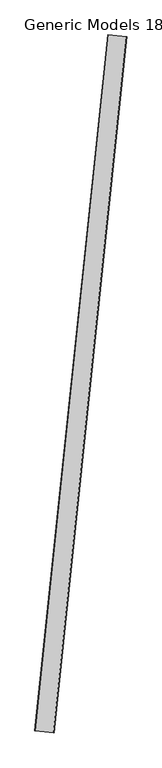
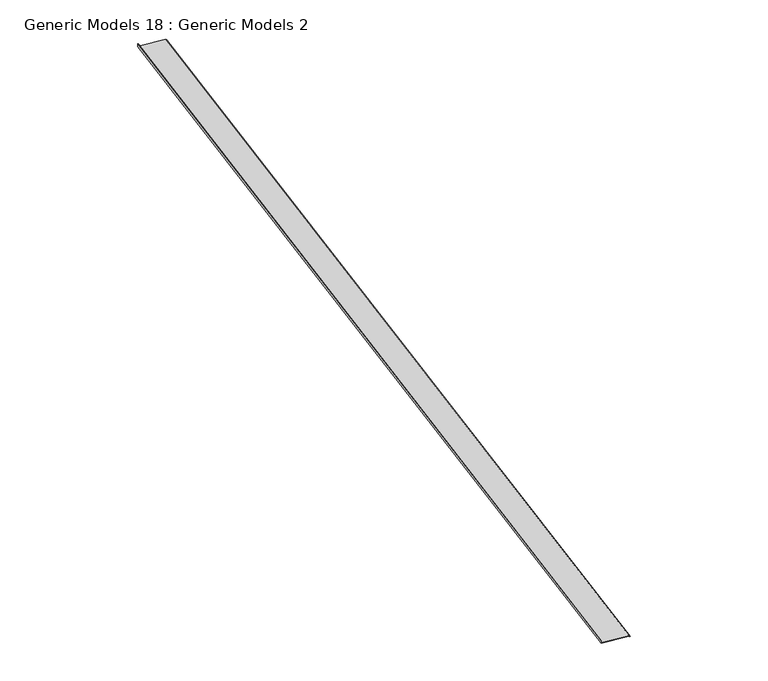
"""IFC4 building model written with IfcOpenShell, lengths in millimetres: proxy geometry, Generic Models 18 : Generic Models 2."""

from ifc_helpers import new_model, si_unit, frame, origin, place, context, project, spatial, polyline, outline, extrude, source, transform, mapped, element, save


def generic_models_18_generic_models_2_1e7d1a4d(model_context):
    return source(origin(), model_context, "Body", "SweptSolid", [
        extrude(outline(polyline([(0.0, 0.0), (1.5875, 0.0), (1.5875, -6.35), (-95.9221094, -103.8596094), (-86.295964, -113.4857549), (-87.418496, -114.6082869), (-98.1671734, -103.8596094), (0.0, -5.692436), (0.0, 0.0)])), frame((33813.0327588, 25672.8767505, 269338.2924407), z_axis=(0.10452846326765233, 0.9945218953682735, 0.0), x_axis=(0.7032331762530428, -0.07391278520352793, 0.7071067811869111)), (0.0, 0.0, 1.0), 5186.9050252),
    ])


if __name__ == "__main__":
    model = new_model("IFC4")
    model_context = context("Model", 3, world=origin())
    ifc_project = project(units=[si_unit("LENGTHUNIT", "METRE", prefix="MILLI")], contexts=[model_context])
    site = spatial("IfcSite", under=ifc_project)
    building = spatial("IfcBuilding", under=site)
    placement = place(None, origin())
    generic_models_18_generic_models_2_shape = generic_models_18_generic_models_2_1e7d1a4d(model_context)
    element("IfcBuildingElementProxy", 1, Name="Generic Models 18 : Generic Models 2", ObjectType="Generic Models 18 : Generic Models 2", at=placement, inside=building, context=model_context, shape_type="MappedRepresentation", body=[
        mapped(generic_models_18_generic_models_2_shape, transform((0.0, 0.0, 0.0), x_axis=(1.0, 0.0, 0.0), y_axis=(0.0, 1.0, 0.0), z_axis=(0.0, 0.0, 1.0))),
    ])
    save(model, "model.ifc")

# Revit data of these elements
# Element 1 (IfcBuildingElementProxy, "Generic Models 18 : Generic Models 2")
#   Materials on its faces: "GALV. BRAKE METAL - (COLOR: GALV.)"
# Materials
#   "GALV. BRAKE METAL - (COLOR: GALV.)": class "Generic", colour RGB 234 234 234, transparency 0, Cost = 0
